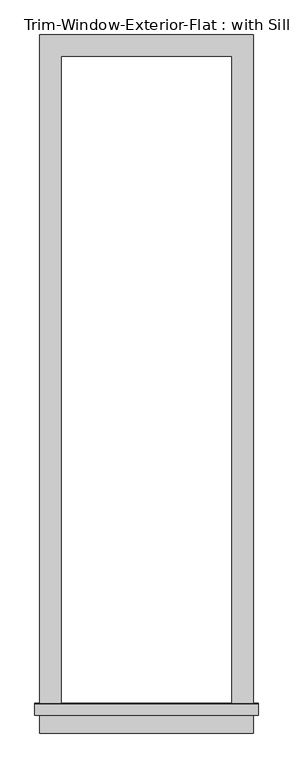
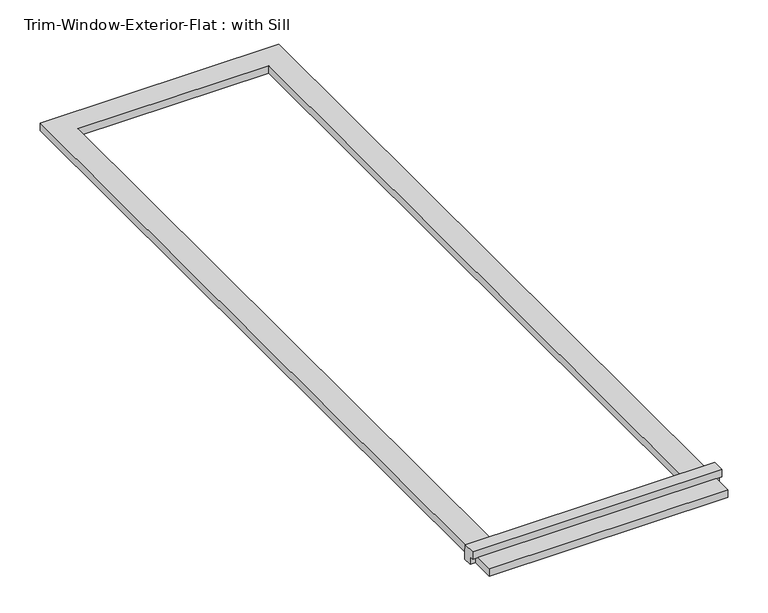
"""IFC4 building model written with IfcOpenShell, lengths in millimetres: proxy geometry, Trim-Window-Exterior-Flat : with Sill."""

import ifcopenshell
import ifcopenshell.guid

model = None  # the IFC model being written
_history = None  # IfcOwnerHistory: only IFC2X3 demands one
_inside = {}  # id of a spatial element -> (the spatial element, [elements in it])
_under = {}  # id of a project, library or spatial element -> (it, [spatial elements below it])
_declared = {}  # id of a project -> (the project, [libraries it declares])
_typed = {}  # id of a type object -> (the type object, [elements of that type])
_made_of = {}  # id of a material, layer set ... -> (it, [elements and type objects made of it])


def new_model(schema):
    """Start an empty IFC model of exactly this schema.

    Asked for "IFC4X3", IfcOpenShell would pick the latest addendum, in which some entities
    have other attributes; the version numbers below select the first issue.
    IFC2X3 requires an IfcOwnerHistory on every rooted entity: one is made here for all.
    """
    global model, _history
    if schema == "IFC4X3":
        model = ifcopenshell.file(schema_version=(4, 3, 0, 0))
    else:
        model = ifcopenshell.file(schema=schema)
    _inside.clear()
    _under.clear()
    _declared.clear()
    _typed.clear()
    _made_of.clear()
    _history = None
    if model.schema == "IFC2X3":
        org = make("IfcOrganization", Name="unknown")
        user = make(
            "IfcPersonAndOrganization",
            ThePerson=make("IfcPerson", FamilyName="unknown"),
            TheOrganization=org,
        )
        app = make(
            "IfcApplication",
            ApplicationDeveloper=org,
            Version="unknown",
            ApplicationFullName="unknown",
            ApplicationIdentifier="unknown",
        )
        _history = make(
            "IfcOwnerHistory",
            OwningUser=user,
            OwningApplication=app,
            ChangeAction="ADDED",
            CreationDate=0,
        )
    return model


def make(cls, **values):
    """One entity of the class cls with the attributes given. An attribute that is None is left unset."""
    return model.create_entity(
        cls, **{name: value for name, value in values.items() if value is not None}
    )


def rooted(cls, **values):
    """An entity with a GlobalId (a new one), such as an element, a storey or a relation."""
    return make(cls, GlobalId=ifcopenshell.guid.new(), OwnerHistory=_history, **values)


def si_unit(unit_type, name, prefix=None):
    """IfcSIUnit, for example si_unit("LENGTHUNIT", "METRE", prefix="MILLI")."""
    return make("IfcSIUnit", UnitType=unit_type, Prefix=prefix, Name=name)


def assignment(units):
    """IfcUnitAssignment: the units of a project."""
    return None if units is None else make("IfcUnitAssignment", Units=units)


def point(xyz):
    """IfcCartesianPoint."""
    return None if xyz is None else make("IfcCartesianPoint", Coordinates=xyz)


def direction(xyz):
    """IfcDirection."""
    return None if xyz is None else make("IfcDirection", DirectionRatios=xyz)


def frame(location, z_axis=None, x_axis=None):
    """IfcAxis2Placement3D, a coordinate frame: its origin and axes. An axis left out is left unset."""
    return make(
        "IfcAxis2Placement3D",
        Location=point(location),
        Axis=direction(z_axis),
        RefDirection=direction(x_axis),
    )


def origin():
    """The frame at (0, 0, 0) with its axes left unset."""
    return frame((0.0, 0.0, 0.0))


def origin_with_axes():
    """The frame at (0, 0, 0) with the z axis (0, 0, 1) and the x axis (1, 0, 0) written out."""
    return frame((0.0, 0.0, 0.0), z_axis=(0.0, 0.0, 1.0), x_axis=(1.0, 0.0, 0.0))


def place(relative_to, where):
    """IfcLocalPlacement: puts the frame where relative to a parent placement (None: the world)."""
    return make(
        "IfcLocalPlacement", PlacementRelTo=relative_to, RelativePlacement=where
    )


def context(
    kind, dimensions, precision=None, world=None, true_north=None, identifier=None
):
    """IfcGeometricRepresentationContext, for example the 3D "Model" context."""
    return make(
        "IfcGeometricRepresentationContext",
        ContextIdentifier=identifier,
        ContextType=kind,
        CoordinateSpaceDimension=dimensions,
        Precision=precision,
        WorldCoordinateSystem=world,
        TrueNorth=true_north,
    )


def project(units=None, contexts=None):
    """IfcProject with its units and contexts."""
    return rooted(
        "IfcProject",
        Name="project",
        RepresentationContexts=contexts,
        UnitsInContext=assignment(units),
    )


def spatial(cls, under=None, at=None, **own):
    """A site, building, storey or space (cls), placed at a placement, below another one or the project."""
    s = rooted(cls, ObjectPlacement=at, **own)
    if under is not None:
        _under.setdefault(under.id(), (under, []))[1].append(s)
    return s


def polyline(points):
    """IfcPolyline through the points."""
    return make("IfcPolyline", Points=[point(p) for p in points])


def outline(outer, holes=None, kind="AREA"):
    """IfcArbitraryClosedProfileDef: a profile drawn as a closed curve; with holes, ...WithVoids."""
    if holes is None:
        return make("IfcArbitraryClosedProfileDef", ProfileType=kind, OuterCurve=outer)
    return make(
        "IfcArbitraryProfileDefWithVoids",
        ProfileType=kind,
        OuterCurve=outer,
        InnerCurves=holes,
    )


def extrude(swept, where, along, depth):
    """IfcExtrudedAreaSolid: the profile swept, set in the frame where, extruded along a direction by depth."""
    return make(
        "IfcExtrudedAreaSolid",
        SweptArea=swept,
        Position=where,
        ExtrudedDirection=direction(along),
        Depth=depth,
    )


def shape(context_of_items, identifier, shape_type, items):
    """IfcShapeRepresentation: the items that make up one representation, for example the "Body"."""
    return make(
        "IfcShapeRepresentation",
        ContextOfItems=context_of_items,
        RepresentationIdentifier=identifier,
        RepresentationType=shape_type,
        Items=items,
    )


def source(mapping_origin, context_of_items, identifier, shape_type, items):
    """IfcRepresentationMap: a shape defined once, which mapped items show again and again."""
    return make(
        "IfcRepresentationMap",
        MappingOrigin=mapping_origin,
        MappedRepresentation=shape(context_of_items, identifier, shape_type, items),
    )


def transform(
    local_origin,
    x_axis=None,
    y_axis=None,
    z_axis=None,
    scale=None,
    scale2=None,
    scale3=None,
    uniform=True,
):
    """IfcCartesianTransformationOperator3D, or its non-uniform kind. x_axis, y_axis, z_axis: its Axis1, 2, 3."""
    if uniform:
        return make(
            "IfcCartesianTransformationOperator3D",
            Axis1=direction(x_axis),
            Axis2=direction(y_axis),
            LocalOrigin=point(local_origin),
            Scale=scale,
            Axis3=direction(z_axis),
        )
    return make(
        "IfcCartesianTransformationOperator3DnonUniform",
        Axis1=direction(x_axis),
        Axis2=direction(y_axis),
        LocalOrigin=point(local_origin),
        Scale=scale,
        Axis3=direction(z_axis),
        Scale2=scale2,
        Scale3=scale3,
    )


def mapped(mapping_source, mapping_target):
    """IfcMappedItem: shows the shape of a source again, moved by a transform."""
    return make(
        "IfcMappedItem", MappingSource=mapping_source, MappingTarget=mapping_target
    )


def made_of(thing, what):
    """Note that an element or type object is made of a material, layer set ...; save() writes the relation."""
    if what is not None:
        _made_of.setdefault(what.id(), (what, []))[1].append(thing)
    return thing


def element(
    cls,
    number,
    at=None,
    inside=None,
    cuts=None,
    type_object=None,
    material=None,
    context=None,
    identifier="Body",
    shape_type=None,
    held_by="IfcProductDefinitionShape",
    body=None,
    shapes=None,
    **own,
):
    """One element of the class cls, such as IfcWall. Its Tag is "e" and its number.

    at: its placement. inside: the storey or other place that contains it. cuts: it is an
    opening in that element (IfcRelVoidsElement). A single representation is given by context,
    identifier, shape_type and body (its items); several are given by shapes. held_by: the class
    of the entity that holds the representations. save() writes the other relations.
    """
    e = rooted(cls, Tag="e%d" % number, ObjectPlacement=at, **own)
    if body is not None:
        shapes = [shape(context, identifier, shape_type, body)]
    if shapes is not None:
        e.Representation = make(held_by, Representations=shapes)
    if inside is not None:
        _inside.setdefault(inside.id(), (inside, []))[1].append(e)
    if cuts is not None:
        rooted(
            "IfcRelVoidsElement", RelatingBuildingElement=cuts, RelatedOpeningElement=e
        )
    if type_object is not None:
        _typed.setdefault(type_object.id(), (type_object, []))[1].append(e)
    return made_of(e, material)


def aggregate(whole, parts):
    """IfcRelAggregates: a whole, such as a stair, and the parts it consists of."""
    return rooted("IfcRelAggregates", RelatingObject=whole, RelatedObjects=parts)


def save(model, path):
    """Write the relations noted so far, then the file.

    IfcRelAggregates (storeys below a building ...), IfcRelContainedInSpatialStructure (elements
    in a storey), IfcRelDefinesByType, IfcRelAssociatesMaterial and IfcRelDeclares: one each for
    every whole, place, type object, material and project.
    """
    for whole, parts in _under.values():
        aggregate(whole, parts)
    for where, things in _inside.values():
        rooted(
            "IfcRelContainedInSpatialStructure",
            RelatedElements=things,
            RelatingStructure=where,
        )
    for kind, things in _typed.values():
        rooted("IfcRelDefinesByType", RelatedObjects=things, RelatingType=kind)
    for what, things in _made_of.values():
        rooted("IfcRelAssociatesMaterial", RelatedObjects=things, RelatingMaterial=what)
    for by, libraries in _declared.values():
        rooted("IfcRelDeclares", RelatingContext=by, RelatedDefinitions=libraries)
    model.write(path)


def trim_window_exterior_flat_with_sill_cd637d81(model_context):
    return source(origin(), model_context, "Body", "SweptSolid", [
        extrude(outline(polyline([(285.75, -1749.3823709), (285.75, -1806.5323709), (-285.75, -1806.5323709), (-285.75, -1749.3823709), (285.75, -1749.3823709)])), origin_with_axes(), (0.0, 0.0, 1.0), 19.05),
        extrude(outline(polyline([(-1758.95, 38.1), (-1729.6580645, 38.1), (-1727.2, 19.05), (-1727.2, 0.0), (-1749.3823709, 0.0), (-1749.3823709, 19.05), (-1758.95, 19.05), (-1758.95, 38.1)])), frame((-298.45, 0.0, 0.0), z_axis=(1.0, 0.0, 0.0), x_axis=(0.0, 1.0, 0.0)), (0.0, 0.0, 1.0), 596.9),
        extrude(outline(polyline([(-285.75, 57.15), (285.75, 57.15), (285.75, -1727.2), (228.6, -1727.2), (228.6, 0.0), (-228.6, 0.0), (-228.6, -1727.2), (-285.75, -1727.2), (-285.75, 57.15)])), origin_with_axes(), (0.0, 0.0, 1.0), 19.05),
    ])


if __name__ == "__main__":
    model = new_model("IFC4")
    model_context = context("Model", 3, world=origin())
    ifc_project = project(units=[si_unit("LENGTHUNIT", "METRE", prefix="MILLI")], contexts=[model_context])
    site = spatial("IfcSite", under=ifc_project)
    building = spatial("IfcBuilding", under=site)
    placement = place(None, origin())
    trim_window_exterior_flat_with_sill_shape = trim_window_exterior_flat_with_sill_cd637d81(model_context)
    element("IfcBuildingElementProxy", 1, Name="Trim-Window-Exterior-Flat : with Sill", ObjectType="Trim-Window-Exterior-Flat : with Sill", at=placement, inside=building, context=model_context, shape_type="MappedRepresentation", body=[
        mapped(trim_window_exterior_flat_with_sill_shape, transform((0.0, 0.0, 0.0), x_axis=(1.0, 0.0, 0.0), y_axis=(0.0, 1.0, 0.0), z_axis=(0.0, 0.0, 1.0))),
    ])
    save(model, "model.ifc")

# Revit data of these elements
# Type "Trim-Window-Exterior-Flat : with Sill"
#   Trim Width = 0' - 2 1/4"
#   Trim Thickness_Picture Frame = 0' - 1 1/4"
#   Trim Thickness_with Sill = 0' - 0 3/4"
#   Sill Thickness = 0' - 1 1/4"
#   Opening Width [instance default] = 2' - 0"
#   Opening Height [instance default] = 3' - 0"
#   Default Elevation = 4' - 0"
#   Sill = yes
#   Picture Frame = no
#   Trim Material [instance default] = none
# Element 1 (IfcBuildingElementProxy, "Trim-Window-Exterior-Flat : with Sill")
#   Opening Width = 1' - 6"
#   Opening Height = 5' - 8"
#   Trim Material = Clad - White
#   Materials on its faces: "Clad - White"
# Materials
#   "Clad - White": class "Wood", colour RGB 242 242 238, transparency 0, Cost = 0
